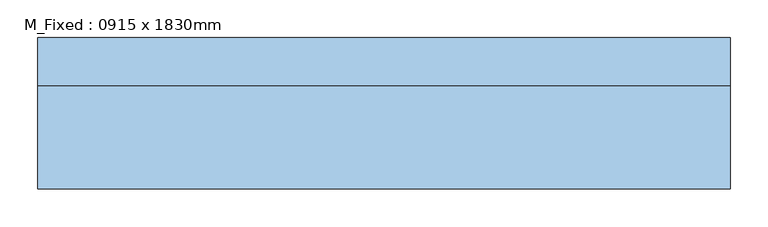
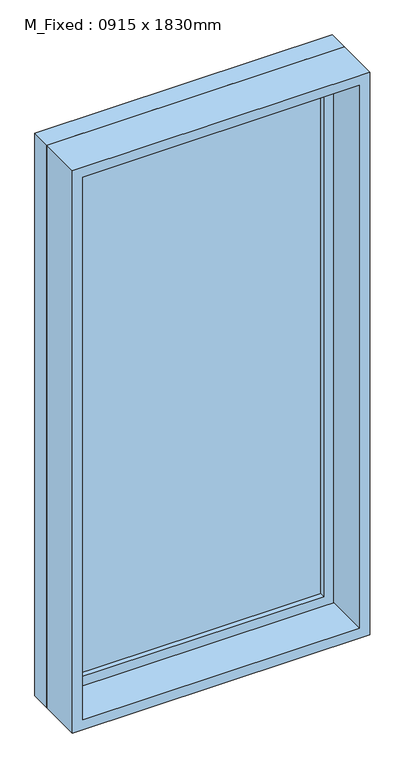
"""IFC4 building model written with IfcOpenShell, lengths in millimetres: window geometry, M_Fixed : 0915 x 1830mm."""

from ifc_helpers import new_model, si_unit, frame, origin, place, context, project, spatial, polyline, outline, extrude, source, transform, mapped, element, save


def m_fixed_0915_x_1830mm_5d6e8bc1(model_context):
    return source(origin(), model_context, "Body", "SweptSolid", [
        extrude(outline(polyline([(-394.5, 78.0), (394.5, 78.0), (394.5, 66.0), (-394.5, 66.0), (-394.5, 78.0)])), frame((0.0, 0.0, 368.0), z_axis=(0.0, 0.0, 1.0), x_axis=(1.0, 0.0, 0.0)), (0.0, 0.0, 1.0), 1704.0),
        extrude(outline(polyline([(2116.0, -438.5), (324.0, -438.5), (324.0, 438.5), (2116.0, 438.5), (2116.0, -438.5)]), holes=[polyline([(2072.0, -394.5), (2072.0, 394.5), (368.0, 394.5), (368.0, -394.5), (2072.0, -394.5)])]), frame((0.0, 50.0, 0.0), z_axis=(0.0, 1.0, 0.0), x_axis=(0.0, 0.0, 1.0)), (0.0, 0.0, 1.0), 44.0),
        extrude(outline(polyline([(2135.0, -457.5), (305.0, -457.5), (305.0, 457.5), (2135.0, 457.5), (2135.0, -457.5)]), holes=[polyline([(2116.0, -438.5), (2116.0, 438.5), (324.0, 438.5), (324.0, -438.5), (2116.0, -438.5)])]), frame((0.0, 50.0, 0.0), z_axis=(0.0, 1.0, 0.0), x_axis=(0.0, 0.0, 1.0)), (0.0, 0.0, 1.0), 63.0),
        extrude(outline(polyline([(2135.0, -457.5), (305.0, -457.5), (305.0, 457.5), (2135.0, 457.5), (2135.0, -457.5)]), holes=[polyline([(2103.0, -425.5), (2103.0, 425.5), (337.0, 425.5), (337.0, -425.5), (2103.0, -425.5)])]), frame((0.0, -87.0, 0.0), z_axis=(0.0, 1.0, 0.0), x_axis=(0.0, 0.0, 1.0)), (0.0, 0.0, 1.0), 137.0),
    ])


if __name__ == "__main__":
    model = new_model("IFC4")
    model_context = context("Model", 3, world=origin())
    ifc_project = project(units=[si_unit("LENGTHUNIT", "METRE", prefix="MILLI")], contexts=[model_context])
    site = spatial("IfcSite", under=ifc_project)
    building = spatial("IfcBuilding", under=site)
    placement = place(None, origin())
    m_fixed_0915_x_1830mm_shape = m_fixed_0915_x_1830mm_5d6e8bc1(model_context)
    element("IfcWindow", 1, ObjectType="M_Fixed : 0915 x 1830mm", at=placement, inside=building, context=model_context, shape_type="MappedRepresentation", body=[
        mapped(m_fixed_0915_x_1830mm_shape, transform((0.0, 0.0, 0.0), x_axis=(1.0, 0.0, 0.0), y_axis=(0.0, 1.0, 0.0), z_axis=(0.0, 0.0, 1.0))),
    ])
    save(model, "model.ifc")

# Revit data of these elements
# Project information
#   Organization Name = "// ORGANIZATION/NAME //"
#   Organization Description = "// ORGANIZATION/DESCRIPTION //"
#   Building Name = "// BUILDING/NAME //"
#   Author = "// AUTHOR //"
#   Project Issue Date = "// ISSUE DATE //"
#   Project Status = "// PROJECT/STATUS //"
#   Client Name = "// CLIENT/NAME //"
#   Project Address = "Enter address here"
#   Project Name = "// PROJECT/NAME //"
#   Project Number = "// PROJECT/NUMBER //"
# Type "M_Fixed : 0915 x 1830mm"
#   Keynote = "Window: Keynote"
#   Model = "Window: Model"
#   Manufacturer = "Window: Manufacturer"
#   URL = "Window: URL"
#   Description = "Window: Description"
#   Assembly Code = "Window: Assembly Code"
#   Type Mark = "Window: Type Mark"
#   Construction Type Id = "GSP4R"
#   Analytic Construction = "1/8 in Pilkington single glazing"
#   Visual Light Transmittance = 0.9
#   Thermal Resistance (R) = 0.271106 (m²·K)/W
#   Solar Heat Gain Coefficient = 0.78
#   Heat Transfer Coefficient (U) = 3.6886 W/(m²·K)
#   Height = 1830 mm
#   Default Sill Height = 305 mm
#   Width = 915 mm
#   Window Inset = 19 mm
#   Define Thermal Properties by = 1
#   Define Thermal Properties by = 1
#   Frame Exterior Material = Sash
#   Frame Interior Material = Sash
#   Glass Pane Material = Glass
#   Sash = Sash
#   Wall Closure = (empty or 0)
# Element 1 (IfcWindow, "M_Fixed : 0915 x 1830mm")
#   Materials on its faces: "Sash", "Glass"
# Materials
#   "Sash": class "Wood", colour RGB 224 178 126, transparency 0, Cost = 0
#   "Glass": class "Glass", colour RGB 0 128 192, transparency 0.9, Description = "Soda Lime Glass", Cost = 0
